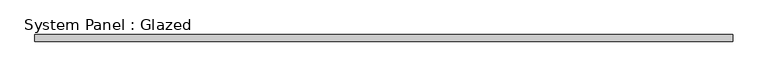
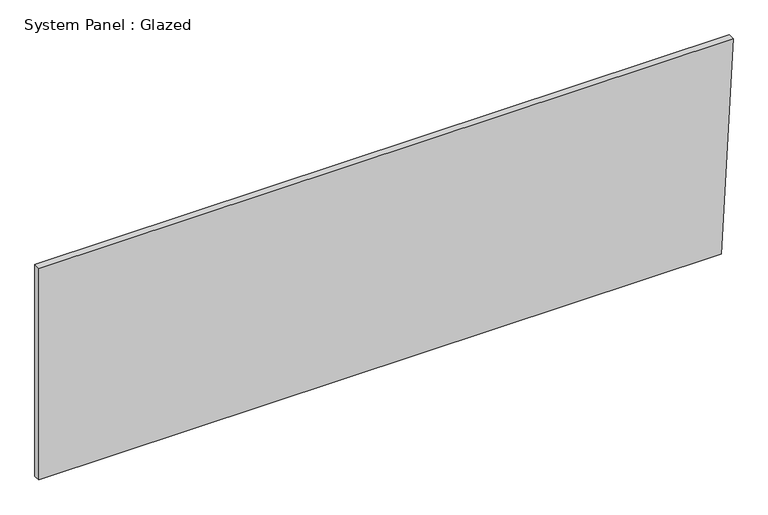
"""IFC4 building model written with IfcOpenShell, lengths in millimetres: plate geometry, System Panel : Glazed."""

from ifc_helpers import new_model, si_unit, frame, origin, place, context, project, spatial, polyline, outline, extrude, source, transform, mapped, element, save


def system_panel_glazed_ef221876(model_context):
    return source(origin(), model_context, "Body", "SweptSolid", [
        extrude(outline(polyline([(0.0, -1343.1943436), (0.0, 1297.8713084), (866.0018549, 1343.1943436), (866.0018549, -1343.1943436), (0.0, -1343.1943436)])), frame((0.0, -44.45, 0.0), z_axis=(0.0, 1.0, 0.0), x_axis=(0.0, 0.0, 1.0)), (0.0, 0.0, 1.0), 25.4),
    ])


if __name__ == "__main__":
    model = new_model("IFC4")
    model_context = context("Model", 3, world=origin())
    ifc_project = project(units=[si_unit("LENGTHUNIT", "METRE", prefix="MILLI")], contexts=[model_context])
    site = spatial("IfcSite", under=ifc_project)
    building = spatial("IfcBuilding", under=site)
    placement = place(None, origin())
    system_panel_glazed_shape = system_panel_glazed_ef221876(model_context)
    element("IfcPlate", 1, ObjectType="System Panel : Glazed", at=placement, inside=building, context=model_context, shape_type="MappedRepresentation", body=[
        mapped(system_panel_glazed_shape, transform((0.0, 0.0, 0.0), x_axis=(1.0, 0.0, 0.0), y_axis=(0.0, 1.0, 0.0), z_axis=(0.0, 0.0, 1.0))),
    ])
    save(model, "model.ifc")

# Revit data of these elements
# Type "System Panel : Glazed"
#   Construction Type Id = "GSP4R"
#   Analytic Construction = "1/8 in Pilkington single glazing"
#   Visual Light Transmittance = 0.9
#   Solar Heat Gain Coefficient = 0.86
#   Heat Transfer Coefficient (U) = 1.18115 BTU/(h·ft²·°F)
#   Define Thermal Properties by = 1
# Element 1 (IfcPlate, "System Panel : Glazed")
#   Materials on its faces: "Glass"
# Materials
#   "Glass": class "Glass", colour RGB 0 128 192, transparency 0.75, Description = "Soda Lime Glass", Cost = 0
